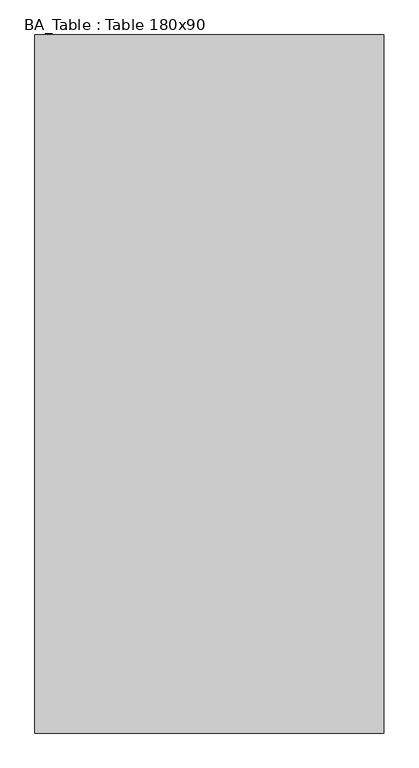
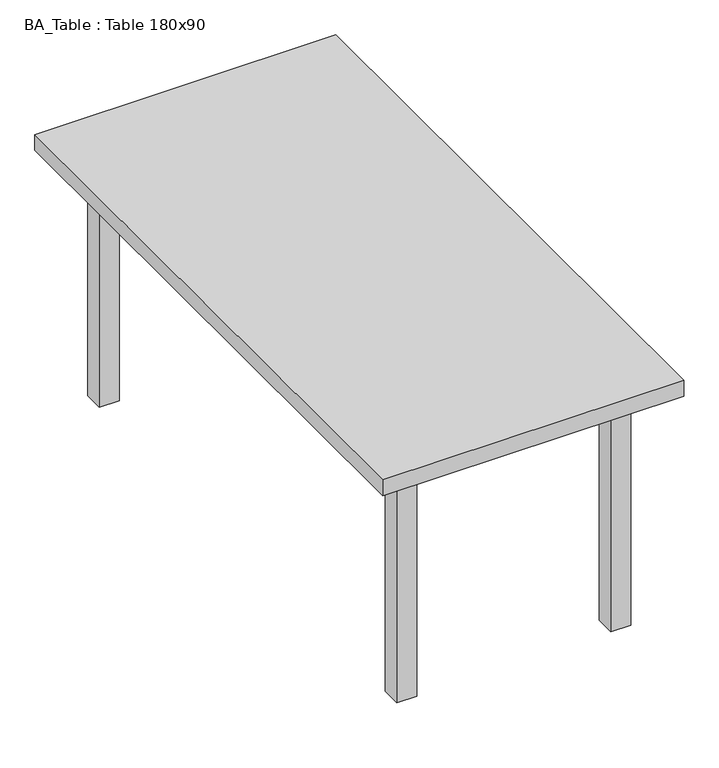
"""IFC4 building model written with IfcOpenShell, lengths in millimetres: furniture geometry, BA_Table : Table 180x90."""

from ifc_helpers import new_model, si_unit, frame, origin, origin_with_axes, place, context, project, spatial, polyline, outline, extrude, source, transform, mapped, element, save


def ba_table_table_180x90_ceb2604b(model_context):
    return source(origin(), model_context, "Body", "SweptSolid", [
        extrude(outline(polyline([(350.0, -740.0), (350.0, -800.0), (290.0, -800.0), (290.0, -740.0), (350.0, -740.0)])), origin_with_axes(), (0.0, 0.0, 1.0), 750.0),
        extrude(outline(polyline([(-290.0, -740.0), (-290.0, -800.0), (-350.0, -800.0), (-350.0, -740.0), (-290.0, -740.0)])), origin_with_axes(), (0.0, 0.0, 1.0), 750.0),
        extrude(outline(polyline([(350.0, 800.0), (350.0, 740.0), (290.0, 740.0), (290.0, 800.0), (350.0, 800.0)])), origin_with_axes(), (0.0, 0.0, 1.0), 750.0),
        extrude(outline(polyline([(-290.0, 800.0), (-290.0, 740.0), (-350.0, 740.0), (-350.0, 800.0), (-290.0, 800.0)])), origin_with_axes(), (0.0, 0.0, 1.0), 750.0),
        extrude(outline(polyline([(450.0, 900.0), (450.0, -900.0), (-450.0, -900.0), (-450.0, 900.0), (450.0, 900.0)])), frame((0.0, 0.0, 750.0), z_axis=(0.0, 0.0, 1.0), x_axis=(1.0, 0.0, 0.0)), (0.0, 0.0, 1.0), 50.0),
    ])


if __name__ == "__main__":
    model = new_model("IFC4")
    model_context = context("Model", 3, world=origin())
    ifc_project = project(units=[si_unit("LENGTHUNIT", "METRE", prefix="MILLI")], contexts=[model_context])
    site = spatial("IfcSite", under=ifc_project)
    building = spatial("IfcBuilding", under=site)
    placement = place(None, origin())
    ba_table_table_180x90_shape = ba_table_table_180x90_ceb2604b(model_context)
    element("IfcFurniture", 1, ObjectType="BA_Table : Table 180x90", at=placement, inside=building, context=model_context, shape_type="MappedRepresentation", body=[
        mapped(ba_table_table_180x90_shape, transform((0.0, 0.0, 0.0), x_axis=(1.0, 0.0, 0.0), y_axis=(0.0, 1.0, 0.0), z_axis=(0.0, 0.0, 1.0))),
    ])
    save(model, "model.ifc")

# Revit data of these elements
# Type "BA_Table : Table 180x90"
#   visina stola = 800 mm
#   sirina stola = 900 mm
#   length = 1800 mm
#   Default Elevation = 0
# Element 1 (IfcFurniture, "BA_Table : Table 180x90")
#   Materials on its faces: "Default"
# Materials
#   "Default": class "Generic", colour RGB 255 255 255, transparency 0, Cost = 0
